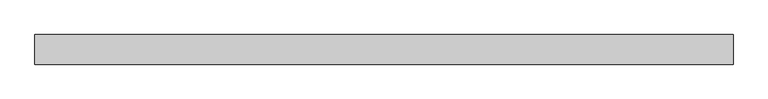
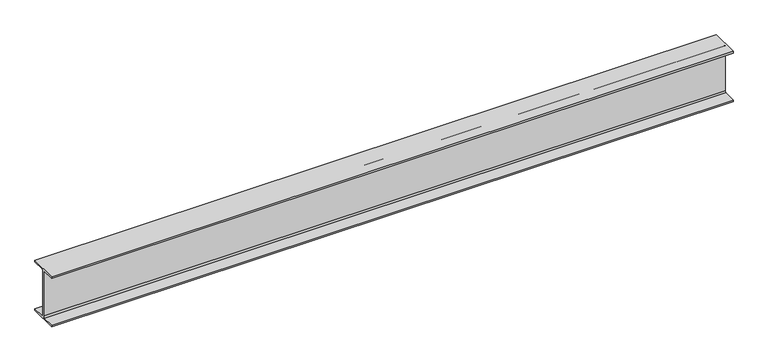
"""IFC4 building model written with IfcOpenShell, lengths in millimetres: beam geometry, Old_Steel Beam_H-KSD3502 : H_SB_ASB_H-250×125x6x9."""

from ifc_helpers import new_model, si_unit, point, frame, frame_2d, origin, place, context, project, spatial, polyline, circle_curve, trimmed, segment, composite_curve, outline, extrude, source, transform, mapped, element, save


def beam_0d167710(model_context):
    return source(origin(), model_context, "Body", "SweptSolid", [
        extrude(outline(composite_curve([segment(polyline([(82.5, -141.5), (82.5, -151.7), (-82.5, -151.7), (-82.5, -141.5), (-11.9, -141.5)]), True, "CONTINUOUS"), segment(trimmed(circle_curve(frame_2d((-11.9, -132.6)), 8.9), [point((-11.9, -141.5))], [point((-3.0, -132.6))], True, "CARTESIAN"), True, "CONTINUOUS"), segment(polyline([(-3.0, -132.6), (-3.0, 132.6)]), True, "CONTINUOUS"), segment(trimmed(circle_curve(frame_2d((-11.9, 132.6)), 8.9), [point((-3.0, 132.6))], [point((-11.9, 141.5))], True, "CARTESIAN"), True, "CONTINUOUS"), segment(polyline([(-11.9, 141.5), (-82.5, 141.5), (-82.5, 151.7), (82.5, 151.7), (82.5, 141.5), (11.9, 141.5)]), True, "CONTINUOUS"), segment(trimmed(circle_curve(frame_2d((11.9, 132.6)), 8.9), [point((11.9, 141.5))], [point((3.0, 132.6))], True, "CARTESIAN"), True, "CONTINUOUS"), segment(polyline([(3.0, 132.6), (3.0, -132.6)]), True, "CONTINUOUS"), segment(trimmed(circle_curve(frame_2d((11.9, -132.6)), 8.9), [point((3.0, -132.6))], [point((11.9, -141.5))], True, "CARTESIAN"), True, "CONTINUOUS"), segment(polyline([(11.9, -141.5), (82.5, -141.5)]), True, "CONTINUOUS")], self_intersect=False)), frame((-1987.2999994, 0.0, 0.0), z_axis=(1.0, 0.0, 0.0), x_axis=(0.0, 1.0, 0.0)), (0.0, 0.0, 1.0), 3892.0999994),
    ])


if __name__ == "__main__":
    model = new_model("IFC4")
    model_context = context("Model", 3, world=origin())
    ifc_project = project(units=[si_unit("LENGTHUNIT", "METRE", prefix="MILLI")], contexts=[model_context])
    site = spatial("IfcSite", under=ifc_project)
    building = spatial("IfcBuilding", under=site)
    placement = place(None, origin())
    beam_shape = beam_0d167710(model_context)
    element("IfcBeam", 1, ObjectType="Old_Steel Beam_H-KSD3502 : H_SB_ASB_H-250×125x6x9", at=placement, inside=building, context=model_context, shape_type="MappedRepresentation", body=[
        mapped(beam_shape, transform((0.0, 0.0, 0.0), x_axis=(1.0, 0.0, 0.0), y_axis=(0.0, 1.0, 0.0), z_axis=(0.0, 0.0, 1.0))),
    ])
    save(model, "model.ifc")

# Revit data of these elements
# Type "Old_Steel Beam_H-KSD3502 : H_SB_ASB_H-250×125x6x9"
#   Width = 12.5 cm
#   Web Thickness = 0.6 cm
#   Web Fillet = 1.2 cm
#   Warping Constant = 42539.8 cm⁶
#   Torsional Moment of Inertia = 7.8102 cm⁴
#   Torsional Modulus = 1.0 cm³
#   Section Area = 37.66 cm²
#   Plastic Modulus weak axis = 73.1 cm³
#   Plastic Modulus strong axis = 366.0 cm³
#   Perimeter = 0.97 m²/m
#   Nominal Weight = 29.60 kgf/m
#   Moment of Inertia weak axis = 294.00 cm⁴
#   Moment of Inertia strong axis = 4050.00 cm⁴
#   Height = 25.0 cm
#   Flange Thickness = 0.9 cm
#   Elastic Modulus weak axis = 47.0 cm³
#   Elastic Modulus strong axis = 324.0 cm³
#   Centroid Vertical = 12.5 cm
#   Centroid Horizontal = 6.25 cm
#   Length [instance default] = 1.5240 m
#   Structural Material [instance default] = Steel, 45-345
#   Assembly Code = ""
# Element 1 (IfcBeam, "Old_Steel Beam_H-KSD3502 : H_SB_ASB_H-250×125x6x9")
#   Structural Material = none
# Materials
#   "Steel, 45-345": class "Metal", colour RGB 189 187 185, transparency 0, Description = "Steel 345 MPa", Cost = 0
